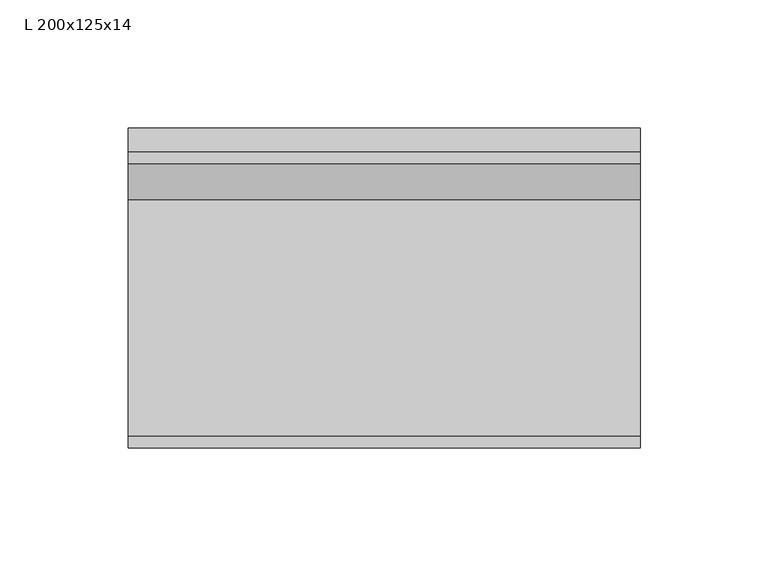
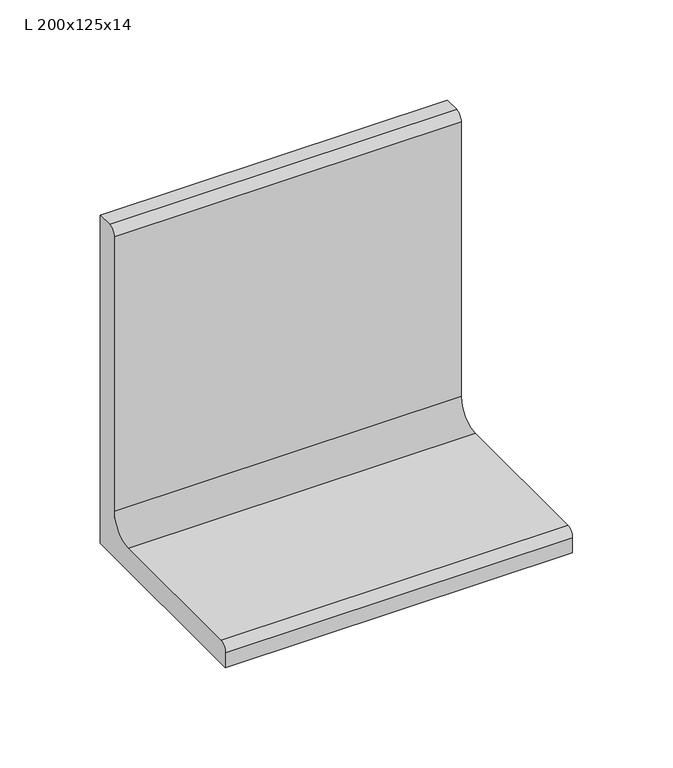
"""IFC4 building model written with IfcOpenShell, lengths in millimetres: beam geometry, Уголок (ГОСТ 8510-86) Балки : L 200x125x14."""

from ifc_helpers import new_model, si_unit, point, frame, frame_2d, origin, place, context, project, spatial, polyline, circle_curve, trimmed, segment, composite_curve, outline, extrude, source, transform, mapped, element, save


def l_200x125x14_c20f8f42(model_context):
    return source(origin(), model_context, "Body", "SweptSolid", [
        extrude(outline(composite_curve([segment(polyline([(29.1, -66.2), (-95.9, -66.2), (-95.9, -56.9)]), True, "CONTINUOUS"), segment(trimmed(circle_curve(frame_2d((-91.2, -56.9)), 4.7), [point((-95.9, -56.9))], [point((-91.2, -52.2))], False, "CARTESIAN"), True, "CONTINUOUS"), segment(polyline([(-91.2, -52.2), (1.1, -52.2)]), True, "CONTINUOUS"), segment(trimmed(circle_curve(frame_2d((1.1, -38.2)), 14.0), [point((1.1, -52.2))], [point((15.1, -38.2))], True, "CARTESIAN"), True, "CONTINUOUS"), segment(polyline([(15.1, -38.2), (15.1, 129.1)]), True, "CONTINUOUS"), segment(trimmed(circle_curve(frame_2d((19.8, 129.1)), 4.7), [point((15.1, 129.1))], [point((19.8, 133.8))], False, "CARTESIAN"), True, "CONTINUOUS"), segment(polyline([(19.8, 133.8), (29.1, 133.8), (29.1, -66.2)]), True, "CONTINUOUS")], self_intersect=False)), frame((-100.0, 0.0, 0.0), z_axis=(1.0, 0.0, 0.0), x_axis=(0.0, 1.0, 0.0)), (0.0, 0.0, 1.0), 200.0),
    ])


if __name__ == "__main__":
    model = new_model("IFC4")
    model_context = context("Model", 3, world=origin())
    ifc_project = project(units=[si_unit("LENGTHUNIT", "METRE", prefix="MILLI")], contexts=[model_context])
    site = spatial("IfcSite", under=ifc_project)
    building = spatial("IfcBuilding", under=site)
    placement = place(None, origin())
    l_200x125x14_shape = l_200x125x14_c20f8f42(model_context)
    element("IfcBeam", 1, ObjectType="Уголок (ГОСТ 8510-86) Балки : L 200x125x14", at=placement, inside=building, context=model_context, shape_type="MappedRepresentation", body=[
        mapped(l_200x125x14_shape, transform((0.0, 0.0, 0.0), x_axis=(1.0, 0.0, 0.0), y_axis=(0.0, 1.0, 0.0), z_axis=(0.0, 0.0, 1.0))),
    ])
    save(model, "model.ifc")

# Revit data of these elements
# Type "Уголок (ГОСТ 8510-86) Балки : L 200x125x14"
#   ri = 4.7 mm
#   ra = 14 mm
#   W = 0.337643
#   Vz = 133.8 mm
#   Vy = 95.9 mm
#   Vpz = 66.2 mm
#   Vpy = 29.1 mm
#   Length [instance default] = 1500 mm
#   bf = 125 mm
#   d = 200 mm
#   tf = 14 mm
#   tw = 14 mm
#   A = 0.004387 m²
#   Structural Material [instance default] = Металл - Сталь - 345 МПa
#   Assembly Code = ""
# Element 1 (IfcBeam, "Уголок (ГОСТ 8510-86) Балки : L 200x125x14")
#   Structural Material = C235
#   Materials on its faces: "C235"
# Materials
#   "Металл - Сталь - 345 МПa": class "Металл", colour RGB 247 247 247, transparency 0
#   "C235": class "Не назначено", colour RGB 0 0 0, transparency 0
